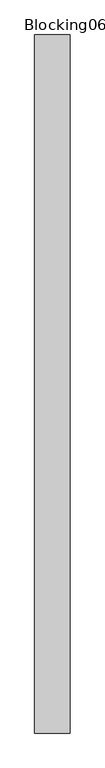
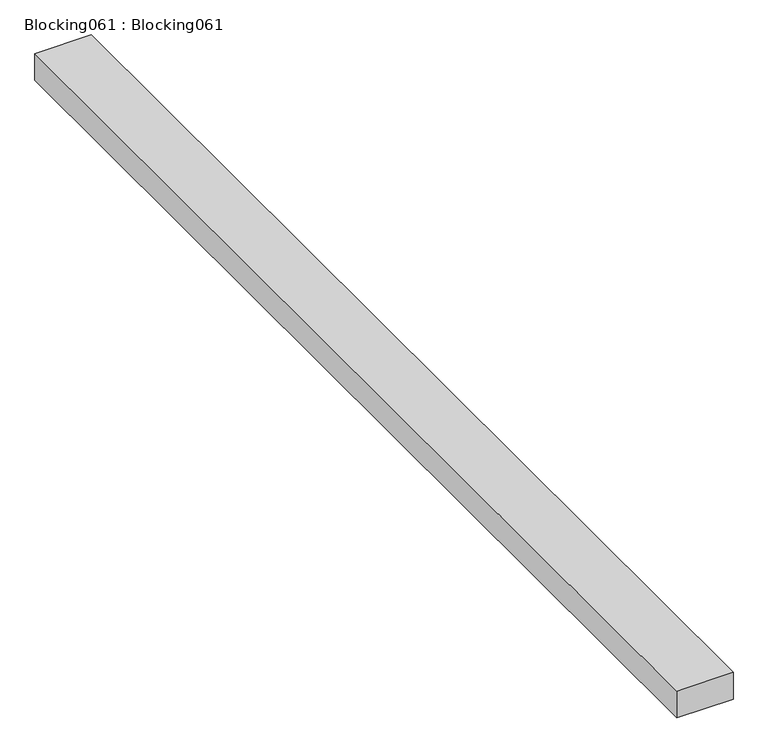
"""IFC4 building model written with IfcOpenShell, lengths in millimetres: proxy geometry, Blocking061 : Blocking061."""

from ifc_helpers import new_model, si_unit, frame, origin, place, context, project, spatial, polyline, outline, extrude, source, transform, mapped, element, save


def blocking061_blocking061_21f17eb5(model_context):
    return source(origin(), model_context, "Body", "SweptSolid", [
        extrude(outline(polyline([(-7121.5276325, 7982.1531721), (-7223.1276325, 7982.1531721), (-7223.1276325, 9982.1531721), (-7121.5276325, 9982.1531721), (-7121.5276325, 7982.1531721)])), frame((0.0, 0.0, 40004.7460083), z_axis=(0.0, 0.0, 1.0), x_axis=(1.0, 0.0, 0.0)), (0.0, 0.0, 1.0), 50.8),
    ])


if __name__ == "__main__":
    model = new_model("IFC4")
    model_context = context("Model", 3, world=origin())
    ifc_project = project(units=[si_unit("LENGTHUNIT", "METRE", prefix="MILLI")], contexts=[model_context])
    site = spatial("IfcSite", under=ifc_project)
    building = spatial("IfcBuilding", under=site)
    placement = place(None, origin())
    blocking061_blocking061_shape = blocking061_blocking061_21f17eb5(model_context)
    element("IfcBuildingElementProxy", 1, Name="Blocking061 : Blocking061", ObjectType="Blocking061 : Blocking061", at=placement, inside=building, context=model_context, shape_type="MappedRepresentation", body=[
        mapped(blocking061_blocking061_shape, transform((0.0, 0.0, 0.0), x_axis=(1.0, 0.0, 0.0), y_axis=(0.0, 1.0, 0.0), z_axis=(0.0, 0.0, 1.0))),
    ])
    save(model, "model.ifc")

# Revit data of these elements
# Type "Blocking061 : Blocking061"
#   NameOverride = "Blocking061"
# Element 1 (IfcBuildingElementProxy, "Blocking061 : Blocking061")
#   Materials on its faces: "WOOD BLOCKING AS REQUIRED"
# Materials
#   "WOOD BLOCKING AS REQUIRED": class "Unassigned", colour RGB 166 124 85, transparency 0, Cost = 0
